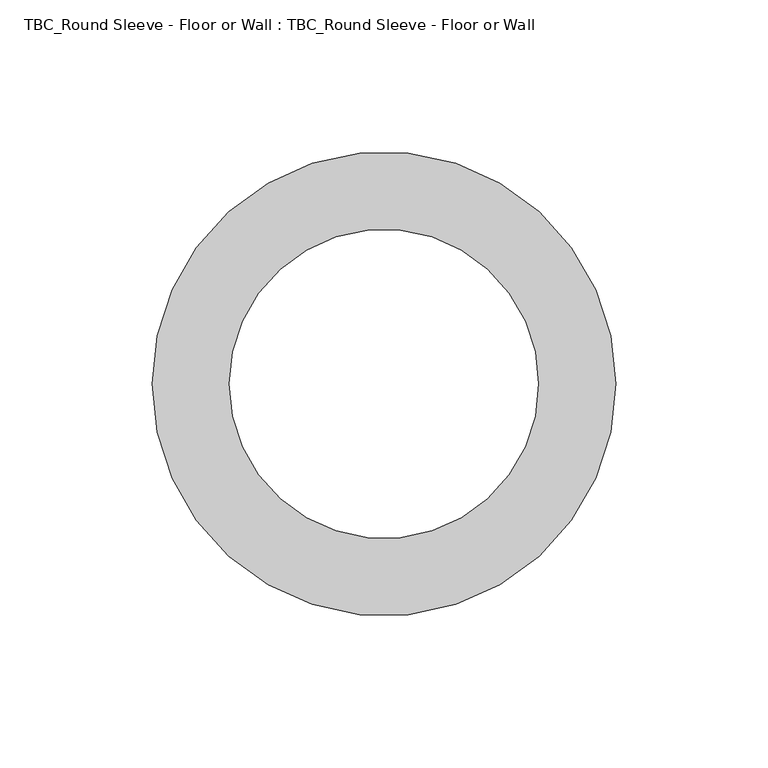
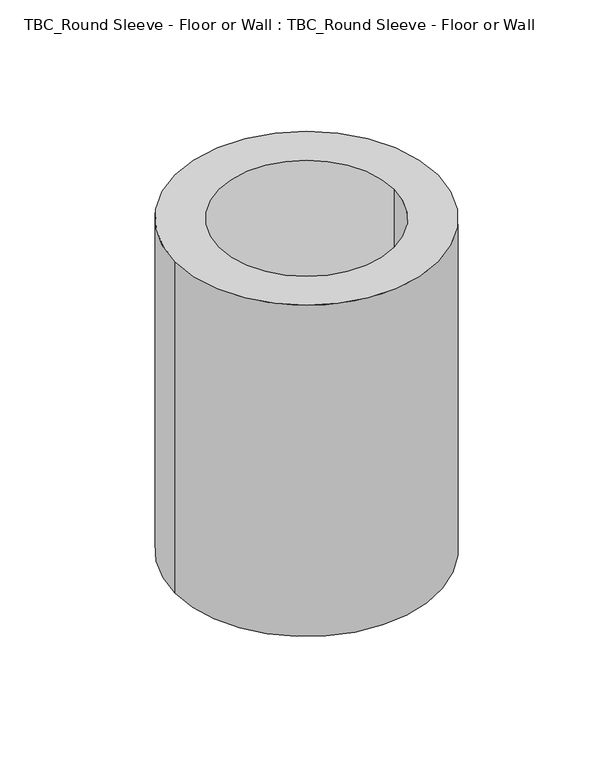
"""IFC4 building model written with IfcOpenShell, lengths in millimetres: proxy geometry, TBC_Round Sleeve - Floor or Wall : TBC_Round Sleeve - Floor or Wall."""

import ifcopenshell
import ifcopenshell.guid

model = None  # the IFC model being written
_history = None  # IfcOwnerHistory: only IFC2X3 demands one
_inside = {}  # id of a spatial element -> (the spatial element, [elements in it])
_under = {}  # id of a project, library or spatial element -> (it, [spatial elements below it])
_declared = {}  # id of a project -> (the project, [libraries it declares])
_typed = {}  # id of a type object -> (the type object, [elements of that type])
_made_of = {}  # id of a material, layer set ... -> (it, [elements and type objects made of it])


def new_model(schema):
    """Start an empty IFC model of exactly this schema.

    Asked for "IFC4X3", IfcOpenShell would pick the latest addendum, in which some entities
    have other attributes; the version numbers below select the first issue.
    IFC2X3 requires an IfcOwnerHistory on every rooted entity: one is made here for all.
    """
    global model, _history
    if schema == "IFC4X3":
        model = ifcopenshell.file(schema_version=(4, 3, 0, 0))
    else:
        model = ifcopenshell.file(schema=schema)
    _inside.clear()
    _under.clear()
    _declared.clear()
    _typed.clear()
    _made_of.clear()
    _history = None
    if model.schema == "IFC2X3":
        org = make("IfcOrganization", Name="unknown")
        user = make(
            "IfcPersonAndOrganization",
            ThePerson=make("IfcPerson", FamilyName="unknown"),
            TheOrganization=org,
        )
        app = make(
            "IfcApplication",
            ApplicationDeveloper=org,
            Version="unknown",
            ApplicationFullName="unknown",
            ApplicationIdentifier="unknown",
        )
        _history = make(
            "IfcOwnerHistory",
            OwningUser=user,
            OwningApplication=app,
            ChangeAction="ADDED",
            CreationDate=0,
        )
    return model


def make(cls, **values):
    """One entity of the class cls with the attributes given. An attribute that is None is left unset."""
    return model.create_entity(
        cls, **{name: value for name, value in values.items() if value is not None}
    )


def rooted(cls, **values):
    """An entity with a GlobalId (a new one), such as an element, a storey or a relation."""
    return make(cls, GlobalId=ifcopenshell.guid.new(), OwnerHistory=_history, **values)


def si_unit(unit_type, name, prefix=None):
    """IfcSIUnit, for example si_unit("LENGTHUNIT", "METRE", prefix="MILLI")."""
    return make("IfcSIUnit", UnitType=unit_type, Prefix=prefix, Name=name)


def assignment(units):
    """IfcUnitAssignment: the units of a project."""
    return None if units is None else make("IfcUnitAssignment", Units=units)


def point(xyz):
    """IfcCartesianPoint."""
    return None if xyz is None else make("IfcCartesianPoint", Coordinates=xyz)


def direction(xyz):
    """IfcDirection."""
    return None if xyz is None else make("IfcDirection", DirectionRatios=xyz)


def frame(location, z_axis=None, x_axis=None):
    """IfcAxis2Placement3D, a coordinate frame: its origin and axes. An axis left out is left unset."""
    return make(
        "IfcAxis2Placement3D",
        Location=point(location),
        Axis=direction(z_axis),
        RefDirection=direction(x_axis),
    )


def frame_2d(location, x_axis=None):
    """IfcAxis2Placement2D, a coordinate frame in the plane: its origin and x axis."""
    return make(
        "IfcAxis2Placement2D", Location=point(location), RefDirection=direction(x_axis)
    )


def origin():
    """The frame at (0, 0, 0) with its axes left unset."""
    return frame((0.0, 0.0, 0.0))


def origin_2d():
    """The frame at (0, 0) in the plane with its x axis left unset."""
    return frame_2d((0.0, 0.0))


def place(relative_to, where):
    """IfcLocalPlacement: puts the frame where relative to a parent placement (None: the world)."""
    return make(
        "IfcLocalPlacement", PlacementRelTo=relative_to, RelativePlacement=where
    )


def context(
    kind, dimensions, precision=None, world=None, true_north=None, identifier=None
):
    """IfcGeometricRepresentationContext, for example the 3D "Model" context."""
    return make(
        "IfcGeometricRepresentationContext",
        ContextIdentifier=identifier,
        ContextType=kind,
        CoordinateSpaceDimension=dimensions,
        Precision=precision,
        WorldCoordinateSystem=world,
        TrueNorth=true_north,
    )


def project(units=None, contexts=None):
    """IfcProject with its units and contexts."""
    return rooted(
        "IfcProject",
        Name="project",
        RepresentationContexts=contexts,
        UnitsInContext=assignment(units),
    )


def spatial(cls, under=None, at=None, **own):
    """A site, building, storey or space (cls), placed at a placement, below another one or the project."""
    s = rooted(cls, ObjectPlacement=at, **own)
    if under is not None:
        _under.setdefault(under.id(), (under, []))[1].append(s)
    return s


def circle_curve(where, radius):
    """IfcCircle in the frame where."""
    return make("IfcCircle", Position=where, Radius=radius)


def trimmed(basis, trim1, trim2, sense, master):
    """IfcTrimmedCurve: the piece of a basis curve between two trims."""
    return make(
        "IfcTrimmedCurve",
        BasisCurve=basis,
        Trim1=trim1,
        Trim2=trim2,
        SenseAgreement=sense,
        MasterRepresentation=master,
    )


def segment(curve, same_sense, transition):
    """IfcCompositeCurveSegment."""
    return make(
        "IfcCompositeCurveSegment",
        Transition=transition,
        SameSense=same_sense,
        ParentCurve=curve,
    )


def composite_curve(segments, self_intersect=None):
    """IfcCompositeCurve: segments joined end to end."""
    return make("IfcCompositeCurve", Segments=segments, SelfIntersect=self_intersect)


def outline(outer, holes=None, kind="AREA"):
    """IfcArbitraryClosedProfileDef: a profile drawn as a closed curve; with holes, ...WithVoids."""
    if holes is None:
        return make("IfcArbitraryClosedProfileDef", ProfileType=kind, OuterCurve=outer)
    return make(
        "IfcArbitraryProfileDefWithVoids",
        ProfileType=kind,
        OuterCurve=outer,
        InnerCurves=holes,
    )


def extrude(swept, where, along, depth):
    """IfcExtrudedAreaSolid: the profile swept, set in the frame where, extruded along a direction by depth."""
    return make(
        "IfcExtrudedAreaSolid",
        SweptArea=swept,
        Position=where,
        ExtrudedDirection=direction(along),
        Depth=depth,
    )


def shape(context_of_items, identifier, shape_type, items):
    """IfcShapeRepresentation: the items that make up one representation, for example the "Body"."""
    return make(
        "IfcShapeRepresentation",
        ContextOfItems=context_of_items,
        RepresentationIdentifier=identifier,
        RepresentationType=shape_type,
        Items=items,
    )


def source(mapping_origin, context_of_items, identifier, shape_type, items):
    """IfcRepresentationMap: a shape defined once, which mapped items show again and again."""
    return make(
        "IfcRepresentationMap",
        MappingOrigin=mapping_origin,
        MappedRepresentation=shape(context_of_items, identifier, shape_type, items),
    )


def transform(
    local_origin,
    x_axis=None,
    y_axis=None,
    z_axis=None,
    scale=None,
    scale2=None,
    scale3=None,
    uniform=True,
):
    """IfcCartesianTransformationOperator3D, or its non-uniform kind. x_axis, y_axis, z_axis: its Axis1, 2, 3."""
    if uniform:
        return make(
            "IfcCartesianTransformationOperator3D",
            Axis1=direction(x_axis),
            Axis2=direction(y_axis),
            LocalOrigin=point(local_origin),
            Scale=scale,
            Axis3=direction(z_axis),
        )
    return make(
        "IfcCartesianTransformationOperator3DnonUniform",
        Axis1=direction(x_axis),
        Axis2=direction(y_axis),
        LocalOrigin=point(local_origin),
        Scale=scale,
        Axis3=direction(z_axis),
        Scale2=scale2,
        Scale3=scale3,
    )


def mapped(mapping_source, mapping_target):
    """IfcMappedItem: shows the shape of a source again, moved by a transform."""
    return make(
        "IfcMappedItem", MappingSource=mapping_source, MappingTarget=mapping_target
    )


def made_of(thing, what):
    """Note that an element or type object is made of a material, layer set ...; save() writes the relation."""
    if what is not None:
        _made_of.setdefault(what.id(), (what, []))[1].append(thing)
    return thing


def element(
    cls,
    number,
    at=None,
    inside=None,
    cuts=None,
    type_object=None,
    material=None,
    context=None,
    identifier="Body",
    shape_type=None,
    held_by="IfcProductDefinitionShape",
    body=None,
    shapes=None,
    **own,
):
    """One element of the class cls, such as IfcWall. Its Tag is "e" and its number.

    at: its placement. inside: the storey or other place that contains it. cuts: it is an
    opening in that element (IfcRelVoidsElement). A single representation is given by context,
    identifier, shape_type and body (its items); several are given by shapes. held_by: the class
    of the entity that holds the representations. save() writes the other relations.
    """
    e = rooted(cls, Tag="e%d" % number, ObjectPlacement=at, **own)
    if body is not None:
        shapes = [shape(context, identifier, shape_type, body)]
    if shapes is not None:
        e.Representation = make(held_by, Representations=shapes)
    if inside is not None:
        _inside.setdefault(inside.id(), (inside, []))[1].append(e)
    if cuts is not None:
        rooted(
            "IfcRelVoidsElement", RelatingBuildingElement=cuts, RelatedOpeningElement=e
        )
    if type_object is not None:
        _typed.setdefault(type_object.id(), (type_object, []))[1].append(e)
    return made_of(e, material)


def aggregate(whole, parts):
    """IfcRelAggregates: a whole, such as a stair, and the parts it consists of."""
    return rooted("IfcRelAggregates", RelatingObject=whole, RelatedObjects=parts)


def save(model, path):
    """Write the relations noted so far, then the file.

    IfcRelAggregates (storeys below a building ...), IfcRelContainedInSpatialStructure (elements
    in a storey), IfcRelDefinesByType, IfcRelAssociatesMaterial and IfcRelDeclares: one each for
    every whole, place, type object, material and project.
    """
    for whole, parts in _under.values():
        aggregate(whole, parts)
    for where, things in _inside.values():
        rooted(
            "IfcRelContainedInSpatialStructure",
            RelatedElements=things,
            RelatingStructure=where,
        )
    for kind, things in _typed.values():
        rooted("IfcRelDefinesByType", RelatedObjects=things, RelatingType=kind)
    for what, things in _made_of.values():
        rooted("IfcRelAssociatesMaterial", RelatedObjects=things, RelatingMaterial=what)
    for by, libraries in _declared.values():
        rooted("IfcRelDeclares", RelatingContext=by, RelatedDefinitions=libraries)
    model.write(path)


def tbc_round_sleeve_floor_or_wall_tbc_round_sleeve_floor_or_f81fbc2f(model_context):
    return source(origin(), model_context, "Body", "SweptSolid", [
        extrude(outline(composite_curve([segment(trimmed(circle_curve(origin_2d(), 76.2), [point((-76.2, 0.0))], [point((76.2, 0.0))], False, "CARTESIAN"), True, "CONTINUOUS"), segment(trimmed(circle_curve(origin_2d(), 76.2), [point((76.2, 0.0))], [point((-76.2, 0.0))], False, "CARTESIAN"), True, "CONTINUOUS")], self_intersect=False), holes=[composite_curve([segment(trimmed(circle_curve(origin_2d(), 50.8), [point((-50.8, 0.0))], [point((50.8, 0.0))], True, "CARTESIAN"), True, "CONTINUOUS"), segment(trimmed(circle_curve(origin_2d(), 50.8), [point((50.8, 0.0))], [point((-50.8, 0.0))], True, "CARTESIAN"), True, "CONTINUOUS")], self_intersect=False)]), frame((0.0, 0.0, -203.2), z_axis=(0.0, 0.0, 1.0), x_axis=(1.0, 0.0, 0.0)), (0.0, 0.0, 1.0), 203.2),
    ])


if __name__ == "__main__":
    model = new_model("IFC4")
    model_context = context("Model", 3, world=origin())
    ifc_project = project(units=[si_unit("LENGTHUNIT", "METRE", prefix="MILLI")], contexts=[model_context])
    site = spatial("IfcSite", under=ifc_project)
    building = spatial("IfcBuilding", under=site)
    placement = place(None, origin())
    tbc_round_sleeve_floor_or_wall_tbc_round_sleeve_floor_or_shape = tbc_round_sleeve_floor_or_wall_tbc_round_sleeve_floor_or_f81fbc2f(model_context)
    element("IfcBuildingElementProxy", 1, Name="TBC_Round Sleeve - Floor or Wall : TBC_Round Sleeve - Floor or Wall", ObjectType="TBC_Round Sleeve - Floor or Wall : TBC_Round Sleeve - Floor or Wall", at=placement, inside=building, context=model_context, shape_type="MappedRepresentation", body=[
        mapped(tbc_round_sleeve_floor_or_wall_tbc_round_sleeve_floor_or_shape, transform((0.0, 0.0, 0.0), x_axis=(1.0, 0.0, 0.0), y_axis=(0.0, 1.0, 0.0), z_axis=(0.0, 0.0, 1.0))),
    ])
    save(model, "model.ifc")

# Revit data of these elements
# Type "TBC_Round Sleeve - Floor or Wall : TBC_Round Sleeve - Floor or Wall"
#   Tag Dimension [instance default] = ""
#   MEP Type [instance default] = ""
#   MEP Element [instance default] = ""
#   MEP Category [instance default] = ""
#   Host Element Type [instance default] = ""
#   Host Element Id [instance default] = ""
#   Host Element Category [instance default] = ""
#   Control Line Y [instance default] = ""
#   Control Line X [instance default] = ""
#   Sleeve Radius [instance default] = 1' - 0"
#   Sleeve Edge [instance default] = 1' - 2"
#   Sleeve Depth [instance default] = 3' - 0"
#   Distance Y [instance default] = 0' - 0"
#   Distance X [instance default] = 0' - 0"
#   Default Elevation = 0
# Element 1 (IfcBuildingElementProxy, "TBC_Round Sleeve - Floor or Wall : TBC_Round Sleeve - Floor or Wall")
#   Tag Dimension = "6\""
#   MEP Type = "PLG-S"
#   MEP Element = "1012458"
#   MEP Category = "Pipe"
#   Host Element Type = "8\" Plank"
#   Host Element Id = "529506"
#   Host Element Category = "Floors"
#   Sleeve Radius = 0' - 4"
#   Sleeve Edge = 0' - 6"
#   Sleeve Depth = 0' - 8"
